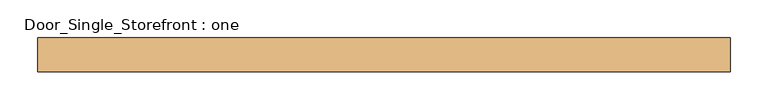
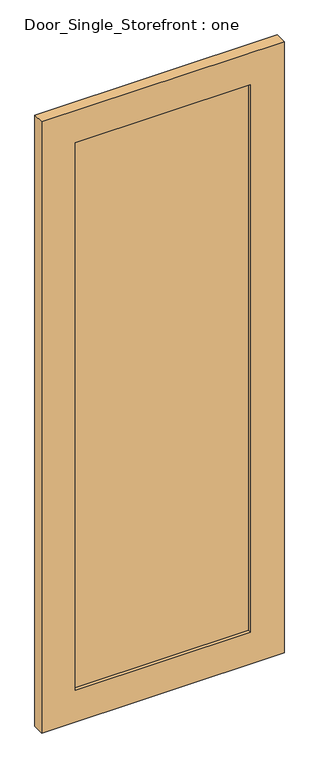
"""IFC4 building model written with IfcOpenShell, lengths in millimetres: door geometry, Door_Single_Storefront : one."""

from ifc_helpers import new_model, si_unit, frame, origin, place, context, project, spatial, polyline, outline, extrude, source, transform, mapped, element, save


def door_single_storefront_one_7f56135a(model_context):
    return source(origin(), model_context, "Body", "SweptSolid", [
        extrude(outline(polyline([(330.2, 6.35), (330.2, -12.7), (-330.2, -12.7), (-330.2, 6.35), (330.2, 6.35)])), frame((0.0, 0.0, 127.0), z_axis=(0.0, 0.0, 1.0), x_axis=(1.0, 0.0, 0.0)), (0.0, 0.0, 1.0), 2184.4),
        extrude(outline(polyline([(2438.4, -457.2), (0.0, -457.2), (0.0, 457.2), (2438.4, 457.2), (2438.4, -457.2)]), holes=[polyline([(127.0, 330.2), (127.0, -330.2), (2311.4, -330.2), (2311.4, 330.2), (127.0, 330.2)])]), frame((0.0, -25.4, 0.0), z_axis=(0.0, 1.0, 0.0), x_axis=(0.0, 0.0, 1.0)), (0.0, 0.0, 1.0), 44.45),
    ])


if __name__ == "__main__":
    model = new_model("IFC4")
    model_context = context("Model", 3, world=origin())
    ifc_project = project(units=[si_unit("LENGTHUNIT", "METRE", prefix="MILLI")], contexts=[model_context])
    site = spatial("IfcSite", under=ifc_project)
    building = spatial("IfcBuilding", under=site)
    placement = place(None, origin())
    door_single_storefront_one_shape = door_single_storefront_one_7f56135a(model_context)
    element("IfcDoor", 1, ObjectType="Door_Single_Storefront : one", at=placement, inside=building, context=model_context, shape_type="MappedRepresentation", body=[
        mapped(door_single_storefront_one_shape, transform((0.0, 0.0, 0.0), x_axis=(1.0, 0.0, 0.0), y_axis=(0.0, 1.0, 0.0), z_axis=(0.0, 0.0, 1.0))),
    ])
    save(model, "model.ifc")

# Revit data of these elements
# Type "Door_Single_Storefront : one"
#   Type Mark = "27"
#   Analytic Construction = "<None>"
#   Stile_Width = 0' - 5"
#   Door_Thickness = 0' - 1 3/4"
#   Door_Offset = 0' - 1"
#   Glass_Material = SAFETY GLAZING
#   Frame_Material = INTERIOR GRADE ALUMINUM STOREFRONT W/ SAFETY GLAZING
#   Function = (empty or 0)
# Element 1 (IfcDoor, "Door_Single_Storefront : one")
#   Materials on its faces: "INTERIOR GRADE ALUMINUM STOREFRONT W/ SAFETY GLAZING", "SAFETY GLAZING"
# Materials
#   "SAFETY GLAZING": class "Glass", colour RGB 142 168 196, transparency 0.75, Description = "Soda Lime Glass", Cost = 0
#   "INTERIOR GRADE ALUMINUM STOREFRONT W/ SAFETY GLAZING": class "Metal", colour RGB 226 226 226, transparency 0, Description = "Aluminum 6061", Cost = 0
